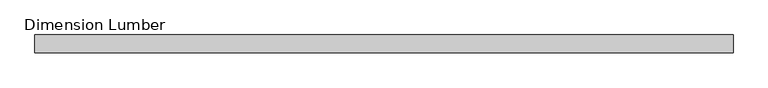
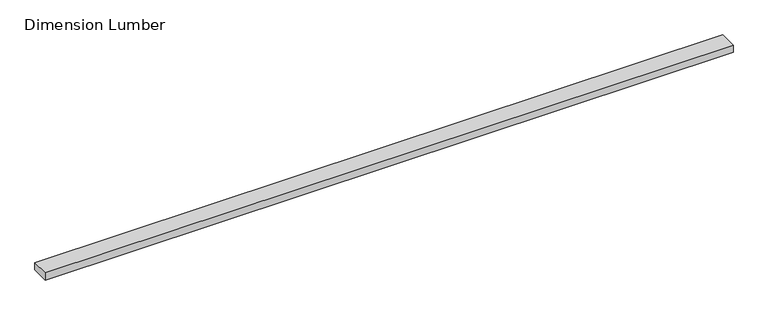
"""IFC4 building model written with IfcOpenShell, lengths in millimetres: beam geometry, Dimension Lumber : Top Supporting Lumbers."""

from ifc_helpers import new_model, si_unit, frame, origin, place, context, project, spatial, polyline, outline, extrude, source, transform, mapped, element, save


def dimension_lumber_dae2390a(model_context):
    return source(origin(), model_context, "Body", "SweptSolid", [
        extrude(outline(polyline([(120.65, 44.45), (120.65, -44.45), (-3333.75, -44.45), (-3333.75, 44.45), (120.65, 44.45)])), frame((0.0, 0.0, -19.05), z_axis=(0.0, 0.0, 1.0), x_axis=(1.0, 0.0, 0.0)), (0.0, 0.0, 1.0), 38.1),
    ])


if __name__ == "__main__":
    model = new_model("IFC4")
    model_context = context("Model", 3, world=origin())
    ifc_project = project(units=[si_unit("LENGTHUNIT", "METRE", prefix="MILLI")], contexts=[model_context])
    site = spatial("IfcSite", under=ifc_project)
    building = spatial("IfcBuilding", under=site)
    placement = place(None, origin())
    dimension_lumber_shape = dimension_lumber_dae2390a(model_context)
    element("IfcBeam", 1, ObjectType="Dimension Lumber : Top Supporting Lumbers", at=placement, inside=building, context=model_context, shape_type="MappedRepresentation", body=[
        mapped(dimension_lumber_shape, transform((0.0, 0.0, 0.0), x_axis=(1.0, 0.0, 0.0), y_axis=(0.0, 1.0, 0.0), z_axis=(0.0, 0.0, 1.0))),
    ])
    save(model, "model.ifc")

# Revit data of these elements
# Type "Dimension Lumber : Top Supporting Lumbers"
#   Assembly Code = "B10"
#   A = 0.0364583 SF
#   Length [instance default] = 5' - 0"
#   b = 0' - 3 1/2"
#   d = 0' - 1 1/2"
#   Structural Material [instance default] = Softwood, Lumber
# Element 1 (IfcBeam, "Dimension Lumber : Top Supporting Lumbers")
#   Structural Material = Douglas Fir #2
#   Materials on its faces: "Douglas Fir #2"
# Materials
#   "Softwood, Lumber": class "Wood", colour RGB 223 192 134, transparency 0, Description = "Pinus Echinata", Cost = 0
#   "Douglas Fir #2": class "Wood", colour RGB 223 192 134, transparency 0, Description = "Pinus Echinata", Cost = 0
